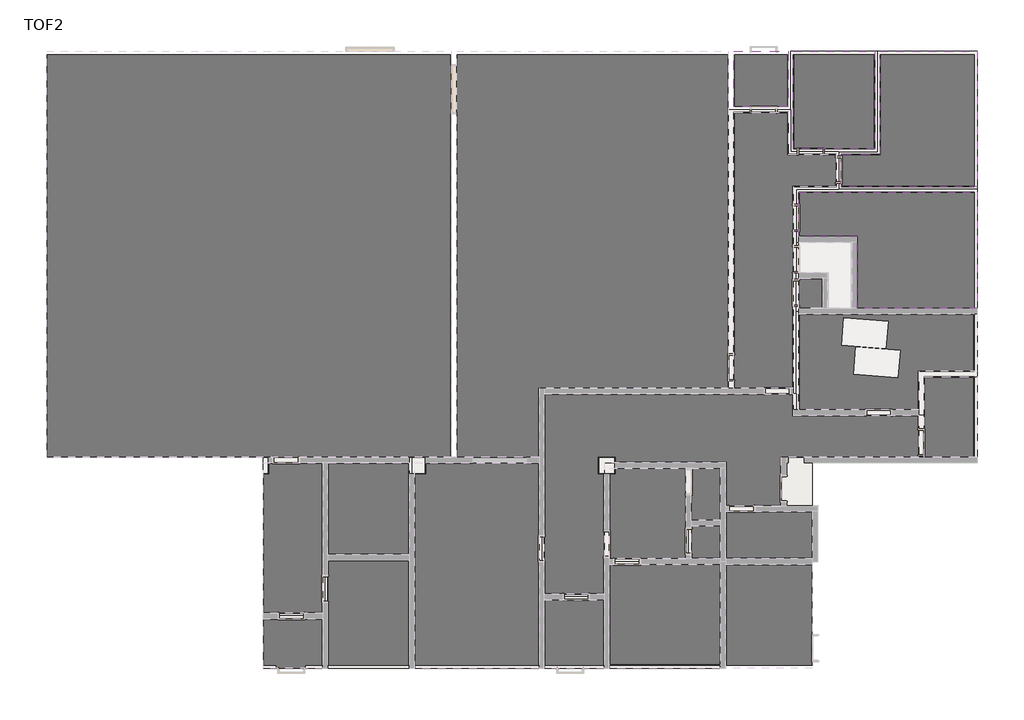
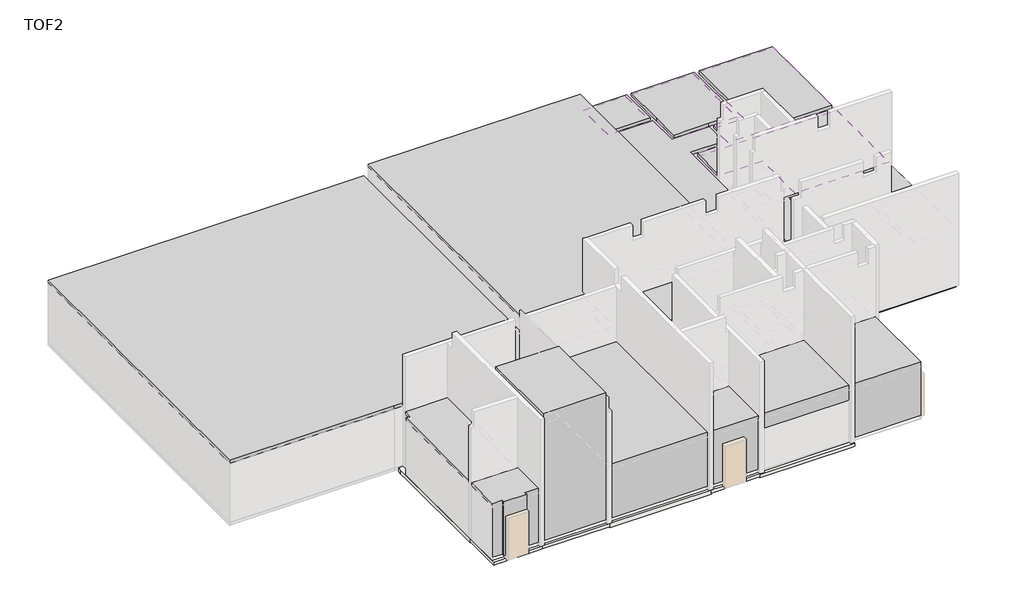
# One storey, part 5 of 5: 24 slabs, 23 proxies, 4 coverings.
# Revit data of these elements (continued)
# Type "H_FL_AR_B07_Vinyl Tile" (continued)
#   Description = ""
#   H_Q'ty Cal Type Tag = "FL-Q1"
#   Function = 0
#   Layers, outside or top first: 7 mm "Vinyl Composition Tile" (function 4)
# Elements 1, 2, 3, 4, 5, 6, 7, 8, 9, 10, 11, 12, 13, 14, 15, 16, 17, 18, 19, 20, 21, 22, 23 (IfcBuildingElementProxy)
#   Comments = "Room Check View Only"
#   Phase Created = New Construction
#   Materials on its faces: "Default"
# Elements 24, 25, 26, 27 (IfcCovering, "H_CE_AR_B09_Acoustic Ceiling_T Bar_600x600x9T")
#   Height Offset From Level = 2700 mm
#   Phase Created = New Construction
# Elements 28, 31, 42, 44, 45 (IfcSlab, "H_SF_AR_S17_SOG T200_GS1")
#   Height Offset From Level = 0 mm
#   Phase Created = New Construction
#   Materials on its faces: "Concrete - Cast-in-Place Concrete - 35 MPa"
# Elements 29, 30, 32, 33, 39 (IfcSlab, "H_SF_AR_S17_SOG T150_GS1")
#   Height Offset From Level = -50 mm
#   Phase Created = New Construction
#   Materials on its faces: "Concrete - Cast-in-Place Concrete - 35 MPa"
# Elements 34, 35, 36, 37, 38, 40, 41, 43, 46 (IfcSlab, "H_SF_AR_S17_SOG T150_GS1")
#   Height Offset From Level = 0 mm
#   Phase Created = New Construction
#   Materials on its faces: "Concrete - Cast-in-Place Concrete - 35 MPa"
# Elements 47, 48, 49, 50, 51 (IfcSlab, "H_FL_AR_B07_Vinyl Tile")
#   Height Offset From Level = 7 mm
#   Phase Created = New Construction
#   Materials on its faces: "Vinyl Composition Tile"
# Materials
#   "Concrete - Cast-in-Place Concrete - 35 MPa": class "Concrete", colour RGB 192 192 192, transparency 0, Description = "ACRYLIC EMULSION PAINT ON THK.13 CEMENT PLASTER", Cost = 0
#   "Vinyl Composition Tile": class "Generic", colour RGB 104 103 102, transparency 0, Description = "Vinyl Composition Tile", Cost = 0
#   "Default": class "Miscellaneous", colour RGB 80 80 80, transparency 0
# Room at (9390, 17931.521) mm, phase "New Construction", upper level "TOC", upper offset 2000 mm, lower offset -1000 mm
#   Comments = ""
#   Number = "101"
#   Name = "MECHANICAL ROOM"
#   H_Floor Finish Style Name = "Non-Slip Epoxy Paint"
#   H_Floor Base Material = "Concrete Slab / Steel Trowel Finish"
#   H_Wall-Base Material-1 = "Masonry Wall"
#   H_Skirt Finish Style Name = "Epoxy Paint"
#   H_Wall-Base Material-2 = ""
#   H_Wall-Base Material-3 = "Plastering"
#   H_Floor-Base Material-1 = "Concrete Slab"
#   H_Floor-Base Material-2 = "Steel Trowel Finish"
#   H_Floor-Base Material-3 = ""
#   H_Floor-Base Material-4 = ""
#   H_Floor-Base Material-5 = ""
#   H_Floor Finish-1 = "Epoxy Paint"
#   H_Floor Finish-2 = ""
#   H_Floor Finish Remark = "*WM 기준 확인 필요 Epoxy Paint \n(용제형, 0.1mm 이하) : epoxy resin + polyamine hardener(경화제)"
#   H_Skirt Base Material = "Same as Wall"
#   H_Skirt-Base Material-1 = ""
#   H_Skirt-Base Material-2 = ""
#   H_Skirt-Base Material-3 = ""
#   H_Skirt-Base Material-4 = ""
#   H_Skirt-Base Material-5 = ""
#   H_Skirt Finish-1 = "Epoxy Paint"
#   H_Skirt Finish-2 = ""
#   H_Skirt Finish Remark = "SACE"
#   H_Wall Finish Style Name = "Acrylic Emulsion Paint"
#   H_Wall Base Material = "Masonry Wall / Cement Plaster"
#   H_Wall-Base Material-4 = ""
#   H_Wall-Base Material-5 = ""
#   H_Wall Finish-1 = "Acrylic Emulsion Paint"
#   H_Wall Finish-2 = ""
#   H_Wall Finish Remark = "T13 Plaster"
#   H_Ceiling Finish Style Name = "Acrylic Emulsion Paint"
#   H_Ceiling Base Material = "Concrete Slab / Fair Faced Concrete"
#   H_Ceiling-Base Material-1 = "(Concrete Slab)"
#   H_Ceiling-Base Material-2 = ""
#   H_Ceiling-Base Material-3 = ""
#   H_Ceiling-Base Material-4 = ""
#   H_Ceiling-Base Material-5 = ""
#   H_Ceiling Finish-1 = "Acrylic Emulsion Paint"
#   H_Ceiling Finish-2 = ""
#   H_Ceiling Finish Remark = "SACE"
#   H_Room W = 17700 mm
#   H_Room L = 11400 mm
#   H_Room H or CH = 7300 mm
#   Floor Finish Style No = F06A
#   Skirt Finish Style No = B03
#   Wall Finish Style No = W01B
#   Ceiling Finish Style No = C01
# Room at (9390, 6347.521) mm, phase "New Construction", upper level "TOC", upper offset 2000 mm, lower offset -1000 mm
#   Comments = ""
#   Number = "112"
#   Name = "ELECTRICAL ROOM(SS08)"
#   H_Floor Finish Style Name = "Non-Slip Epoxy Paint"
#   H_Floor Base Material = "Concrete Slab / Screed"
#   H_Wall-Base Material-1 = "Masonry Wall"
#   H_Skirt Finish Style Name = "Epoxy Paint"
#   H_Wall-Base Material-2 = ""
#   H_Wall-Base Material-3 = "Plastering"
#   H_Floor-Base Material-1 = "Concrete Slab"
#   H_Floor-Base Material-2 = ""
#   H_Floor-Base Material-3 = "Screed"
#   H_Floor-Base Material-4 = ""
#   H_Floor-Base Material-5 = ""
#   H_Floor Finish-1 = "Epoxy Paint"
#   H_Floor Finish-2 = ""
#   H_Floor Finish Remark = "*WM 기준 확인 필요 Epoxy Paint \n(용제형, 0.1mm 이하) : epoxy resin + polyamine hardener(경화제)"
#   H_Skirt Base Material = "Same as Wall"
#   H_Skirt-Base Material-1 = ""
#   H_Skirt-Base Material-2 = ""
#   H_Skirt-Base Material-3 = ""
#   H_Skirt-Base Material-4 = ""
#   H_Skirt-Base Material-5 = ""
#   H_Skirt Finish-1 = "Epoxy Paint"
#   H_Skirt Finish-2 = ""
#   H_Skirt Finish Remark = "SACE"
#   H_Wall Finish Style Name = "Acrylic Emulsion Paint"
#   H_Wall Base Material = "Masonry Wall / Cement Plaster"
#   H_Wall-Base Material-4 = ""
#   H_Wall-Base Material-5 = ""
#   H_Wall Finish-1 = "Acrylic Emulsion Paint"
#   H_Wall Finish-2 = ""
#   H_Wall Finish Remark = "T13 Plaster"
#   H_Ceiling Finish Style Name = "Acrylic Emulsion Paint"
#   H_Ceiling Base Material = "Concrete Slab / Fair Faced Concrete"
#   H_Ceiling-Base Material-1 = "(Concrete Slab)"
#   H_Ceiling-Base Material-2 = ""
#   H_Ceiling-Base Material-3 = ""
#   H_Ceiling-Base Material-4 = ""
#   H_Ceiling-Base Material-5 = ""
#   H_Ceiling Finish-1 = "Acrylic Emulsion Paint"
#   H_Ceiling Finish-2 = ""
#   H_Ceiling Finish Remark = "SACE"
#   H_Room W = 17700 mm
#   H_Room L = 11000 mm
#   H_Room H or CH = 7300 mm
#   Floor Finish Style No = F06B
#   Skirt Finish Style No = B03
#   Wall Finish Style No = W01B
#   Ceiling Finish Style No = C01
# Room at (25850, 15981.521) mm, phase "New Construction", upper level "TOC", upper offset 2000 mm, lower offset 0 mm
#   Comments = ""
#   Number = "102"
#   Name = "RACK ROOM"
#   H_Floor Finish Style Name = "Anti-Dust Epoxy Paint / Anti-Static Vinyl Tile on Raised Floor"
#   H_Floor Base Material = "Concrete Slab / Steel Trowel Finish"
#   H_Wall-Base Material-1 = "Masonry Wall"
#   H_Skirt Finish Style Name = "Coved Vinyl Tile"
#   H_Wall-Base Material-2 = ""
#   H_Wall-Base Material-3 = "Plastering"
#   H_Floor-Base Material-1 = "Concrete Slab"
#   H_Floor-Base Material-2 = "Steel Trowel Finish"
#   H_Floor-Base Material-3 = ""
#   H_Floor-Base Material-4 = ""
#   H_Floor-Base Material-5 = "Raised Floor_Anti-Static Vinyl Tile"
#   H_Floor Finish-1 = "Anti-Dust Paint"
#   H_Floor Finish-2 = "Raised Floor_Anti-Static Vinyl Tile"
#   H_Floor Finish Remark = "600x600, H=1000"
#   H_Skirt Base Material = "Same as Wall"
#   H_Skirt-Base Material-1 = ""
#   H_Skirt-Base Material-2 = ""
#   H_Skirt-Base Material-3 = ""
#   H_Skirt-Base Material-4 = ""
#   H_Skirt-Base Material-5 = ""
#   H_Skirt Finish-1 = "Vinyl Tile"
#   H_Skirt Finish-2 = ""
#   H_Skirt Finish Remark = "Vinyl Tile = PVC Tile (polyvinyl chloride)"
#   H_Wall Finish Style Name = "Acrylic Emulsion Paint"
#   H_Wall Base Material = "Masonry Wall / Cement Plaster"
#   H_Wall-Base Material-4 = ""
#   H_Wall-Base Material-5 = ""
#   H_Wall Finish-1 = "Acrylic Emulsion Paint"
#   H_Wall Finish-2 = ""
#   H_Wall Finish Remark = "T13 Plaster"
#   H_Ceiling Finish Style Name = "Suspended Acoustic Tiled Ceiling (M-Bar)"
#   H_Ceiling Base Material = "Concrete Slab / Fair Faced Concrete"
#   H_Ceiling-Base Material-1 = "(Concrete Slab)"
#   H_Ceiling-Base Material-2 = "(Fair Faced Concrete)"
#   H_Ceiling-Base Material-3 = ""
#   H_Ceiling-Base Material-4 = ""
#   H_Ceiling-Base Material-5 = "Acoustic Tiled Ceiling System (M-Bar)"
#   H_Ceiling Finish-1 = "Acoustic Tiled Ceiling System (M-Bar)"
#   H_Ceiling Finish-2 = ""
#   H_Ceiling Finish Remark = ""
#   H_Room W = 14900 mm
#   H_Room L = 14900 mm
#   H_Room H or CH = 3000 mm
#   Floor Finish Style No = F91
#   Skirt Finish Style No = B35
#   Wall Finish Style No = W01B
#   Ceiling Finish Style No = C95A
# Room at (22100, 4784.521) mm, phase "New Construction", upper level "TOC", upper offset 2000 mm, lower offset -1000 mm
#   Comments = ""
#   Number = "114"
#   Name = "BATTERY ROOM"
#   H_Floor Finish Style Name = "Acid Resistant Ceramic Tile"
#   H_Floor Base Material = "Concrete Slab / Steel Trowel Finish"
#   H_Wall-Base Material-1 = "Masonry Wall"
#   H_Skirt Finish Style Name = "Coved Vinyl Tile"
#   H_Wall-Base Material-2 = ""
#   H_Wall-Base Material-3 = "Plastering"
#   H_Floor-Base Material-1 = "Concrete Slab"
#   H_Floor-Base Material-2 = "Steel Trowel Finish"
#   H_Floor-Base Material-3 = ""
#   H_Floor-Base Material-4 = ""
#   H_Floor-Base Material-5 = "Acid/Alkaline Resistant Tile"
#   H_Floor Finish-1 = "Acid/Alkaline Resistant Tile"
#   H_Floor Finish-2 = ""
#   H_Floor Finish Remark = "*WM : Bonding용 Mortar은 Tile에 포함\n*Slope 용 Screed만 별도 구분 (Concrete 바닥 단차 발생하는 경우 Only)"
#   H_Skirt Base Material = "Same as Wall"
#   H_Skirt-Base Material-1 = ""
#   H_Skirt-Base Material-2 = ""
#   H_Skirt-Base Material-3 = ""
#   H_Skirt-Base Material-4 = ""
#   H_Skirt-Base Material-5 = ""
#   H_Skirt Finish-1 = "Vinyl Tile"
#   H_Skirt Finish-2 = ""
#   H_Skirt Finish Remark = "Vinyl Tile = PVC Tile (polyvinyl chloride)"
#   H_Wall Finish Style Name = "Acid Resistant Paint"
#   H_Wall Base Material = "Masonry Wall / Cement Plaster"
#   H_Wall-Base Material-4 = ""
#   H_Wall-Base Material-5 = ""
#   H_Wall Finish-1 = "Acid/Alkaline Resistant Paint"
#   H_Wall Finish-2 = ""
#   H_Wall Finish Remark = "T13 Plaster"
#   H_Ceiling Finish Style Name = "Acrylic Emulsion Paint"
#   H_Ceiling Base Material = "Concrete Slab / Fair Faced Concrete"
#   H_Ceiling-Base Material-1 = "(Concrete Slab)"
#   H_Ceiling-Base Material-2 = ""
#   H_Ceiling-Base Material-3 = ""
#   H_Ceiling-Base Material-4 = ""
#   H_Ceiling-Base Material-5 = ""
#   H_Ceiling Finish-1 = "Acrylic Emulsion Paint"
#   H_Ceiling Finish-2 = ""
#   H_Ceiling Finish Remark = "SACE"
#   H_Room W = 7700 mm
#   H_Room L = 7500 mm
#   H_Room H or CH = 7300 mm
#   Floor Finish Style No = F32A
#   Skirt Finish Style No = B35
#   Wall Finish Style No = W04B
#   Ceiling Finish Style No = C01
# Room at (34305, 4784.521) mm, phase "New Construction", upper level "TOC", upper offset 2000 mm, lower offset 0 mm
#   Comments = ""
#   Number = "118"
#   Name = "DRIVERS LOUNGE"
#   H_Floor Finish Style Name = "Vinyl Tile"
#   H_Floor Base Material = "Concrete Slab / Steel Trowel Finish"
#   H_Wall-Base Material-1 = "Masonry Wall"
#   H_Skirt Finish Style Name = "Coved Vinyl Tile"
#   H_Wall-Base Material-2 = ""
#   H_Wall-Base Material-3 = "Plastering"
#   H_Floor-Base Material-1 = "Concrete Slab"
#   H_Floor-Base Material-2 = "Steel Trowel Finish"
#   H_Floor-Base Material-3 = ""
#   H_Floor-Base Material-4 = ""
#   H_Floor-Base Material-5 = "Vinyl Tile"
#   H_Floor Finish-1 = "Vinyl Tile"
#   H_Floor Finish-2 = ""
#   H_Floor Finish Remark = ""
#   H_Skirt Base Material = "Same as Wall"
#   H_Skirt-Base Material-1 = ""
#   H_Skirt-Base Material-2 = ""
#   H_Skirt-Base Material-3 = ""
#   H_Skirt-Base Material-4 = ""
#   H_Skirt-Base Material-5 = ""
#   H_Skirt Finish-1 = "Vinyl Tile"
#   H_Skirt Finish-2 = ""
#   H_Skirt Finish Remark = "Vinyl Tile = PVC Tile (polyvinyl chloride)"
#   H_Wall Finish Style Name = "Acrylic Emulsion Paint"
#   H_Wall Base Material = "Masonry Wall / Cement Plaster"
#   H_Wall-Base Material-4 = ""
#   H_Wall-Base Material-5 = ""
#   H_Wall Finish-1 = "Acrylic Emulsion Paint"
#   H_Wall Finish-2 = ""
#   H_Wall Finish Remark = "T13 Plaster"
#   H_Ceiling Finish Style Name = "Suspended Acoustic Tiled Ceiling (M-Bar)"
#   H_Ceiling Base Material = "Concrete Slab / Fair Faced Concrete"
#   H_Ceiling-Base Material-1 = "(Concrete Slab)"
#   H_Ceiling-Base Material-2 = "(Fair Faced Concrete)"
#   H_Ceiling-Base Material-3 = ""
#   H_Ceiling-Base Material-4 = ""
#   H_Ceiling-Base Material-5 = "Acoustic Tiled Ceiling System (M-Bar)"
#   H_Ceiling Finish-1 = "Acoustic Tiled Ceiling System (M-Bar)"
#   H_Ceiling Finish-2 = ""
#   H_Ceiling Finish Remark = ""
#   H_Room W = 4500 mm
#   H_Room L = 7500 mm
#   H_Room H or CH = 2600 mm
#   Floor Finish Style No = F34A
#   Skirt Finish Style No = B35
#   Wall Finish Style No = W01B
#   Ceiling Finish Style No = C95A
# Room at (38540.953, 16104.521) mm, phase "New Construction", upper level "TOC", upper offset 2000 mm, lower offset 0 mm
#   Comments = ""
#   Number = "103"
#   Name = "CONTROL ROOM"
#   H_Floor Finish Style Name = "Anti-Dust Epoxy Paint / Anti-Static Vinyl Tile on Raised Floor"
#   H_Floor Base Material = "Concrete Slab / Steel Trowel Finish"
#   H_Wall-Base Material-1 = "Masonry Wall"
#   H_Skirt Finish Style Name = "Coved Vinyl Tile"
#   H_Wall-Base Material-2 = ""
#   H_Wall-Base Material-3 = "Plastering"
#   H_Floor-Base Material-1 = "Concrete Slab"
#   H_Floor-Base Material-2 = "Steel Trowel Finish"
#   H_Floor-Base Material-3 = ""
#   H_Floor-Base Material-4 = ""
#   H_Floor-Base Material-5 = "Raised Floor_Anti-Static Vinyl Tile"
#   H_Floor Finish-1 = "Anti-Dust Paint"
#   H_Floor Finish-2 = "Raised Floor_Anti-Static Vinyl Tile"
#   H_Floor Finish Remark = "600x600, H=1000"
#   H_Skirt Base Material = "Same as Wall"
#   H_Skirt-Base Material-1 = ""
#   H_Skirt-Base Material-2 = ""
#   H_Skirt-Base Material-3 = ""
#   H_Skirt-Base Material-4 = ""
#   H_Skirt-Base Material-5 = ""
#   H_Skirt Finish-1 = "Vinyl Tile"
#   H_Skirt Finish-2 = ""
#   H_Skirt Finish Remark = "Vinyl Tile = PVC Tile (polyvinyl chloride)"
#   H_Wall Finish Style Name = "Acrylic Emulsion Paint"
#   H_Wall Base Material = "Masonry Wall / Cement Plaster"
#   H_Wall-Base Material-4 = ""
#   H_Wall-Base Material-5 = ""
#   H_Wall Finish-1 = "Acrylic Emulsion Paint"
#   H_Wall Finish-2 = ""
#   H_Wall Finish Remark = "T13 Plaster"
#   H_Ceiling Finish Style Name = "Suspended Acoustic Tiled Ceiling (M-Bar)"
#   H_Ceiling Base Material = "Concrete Slab / Fair Faced Concrete"
#   H_Ceiling-Base Material-1 = "(Concrete Slab)"
#   H_Ceiling-Base Material-2 = "(Fair Faced Concrete)"
#   H_Ceiling-Base Material-3 = ""
#   H_Ceiling-Base Material-4 = ""
#   H_Ceiling-Base Material-5 = "Acoustic Tiled Ceiling System (M-Bar)"
#   H_Ceiling Finish-1 = "Acoustic Tiled Ceiling System (M-Bar)"
#   H_Ceiling Finish-2 = ""
#   H_Ceiling Finish Remark = ""
#   H_Room W = 10000 mm
#   H_Room L = 14900 mm
#   H_Room H or CH = 3500 mm
#   Floor Finish Style No = F91
#   Skirt Finish Style No = B35
#   Wall Finish Style No = W01B
#   Ceiling Finish Style No = C95A
# Room at (41150, 2419.673) mm, phase "New Construction", upper level "TOC", upper offset 2000 mm, lower offset 0 mm
#   Comments = ""
#   Number = "122"
#   Name = "TOILETS"
#   H_Floor Finish Style Name = "Non-Slip Unglazed Ceramic Tile"
#   H_Floor Base Material = "Concrete Slab / Screed / Liquid Waterproofing"
#   H_Wall-Base Material-1 = "Masonry Wall"
#   H_Skirt Finish Style Name = "Coved Ceramic Tile"
#   H_Wall-Base Material-2 = ""
#   H_Wall-Base Material-3 = ""
#   H_Floor-Base Material-1 = "Concrete Slab"
#   H_Floor-Base Material-2 = ""
#   H_Floor-Base Material-3 = "Screed"
#   H_Floor-Base Material-4 = "Liquid Waterproofing"
#   H_Floor-Base Material-5 = "Ceramic Tile"
#   H_Floor Finish-1 = "Ceramic Tile"
#   H_Floor Finish-2 = ""
#   H_Floor Finish Remark = ""
#   H_Skirt Base Material = "Same as Wall"
#   H_Skirt-Base Material-1 = ""
#   H_Skirt-Base Material-2 = ""
#   H_Skirt-Base Material-3 = ""
#   H_Skirt-Base Material-4 = ""
#   H_Skirt-Base Material-5 = ""
#   H_Skirt Finish-1 = "Glazed Ceramic Tile"
#   H_Skirt Finish-2 = ""
#   H_Skirt Finish Remark = ""
#   H_Wall Finish Style Name = "Glazed Ceramic Tile (≤C.H+100) / No Paint (>C.H+100)"
#   H_Wall Base Material = "Masonry Wall / Liquid Waterproofing"
#   H_Wall-Base Material-4 = "Liquid Waterproofing"
#   H_Wall-Base Material-5 = "Glazed Ceramic Tile"
#   H_Wall Finish-1 = "Glazed Ceramic Tile"
#   H_Wall Finish-2 = ""
#   H_Wall Finish Remark = "Below Suspended Ceiling\nGlazed Ceramic Tile(≤C.H+100) + Liquid Waterproofing / No Paint (>C.H+100)"
#   H_Ceiling Finish Style Name = "Suspended Moisture Resistant Tiled Ceiling (M-Bar)"
#   H_Ceiling Base Material = "Concrete Slab / Fair Faced Concrete"
#   H_Ceiling-Base Material-1 = "(Concrete Slab)"
#   H_Ceiling-Base Material-2 = "(Fair Faced Concrete)"
#   H_Ceiling-Base Material-3 = ""
#   H_Ceiling-Base Material-4 = ""
#   H_Ceiling-Base Material-5 = "Moisture Resistant Tiled Ceiling System (M-Bar)"
#   H_Ceiling Finish-1 = "Moisture Resistant Tiled Ceiling System (M-Bar)"
#   H_Ceiling Finish-2 = ""
#   H_Ceiling Finish Remark = ""
#   H_Room W = 4000 mm
#   H_Room L = 3700 mm
#   H_Room H or CH = 2600 mm
#   Floor Finish Style No = F31B
#   Skirt Finish Style No = B32
#   Wall Finish Style No = W32B
#   Ceiling Finish Style No = C96A
# Room at (49742.5, 4429.521) mm, phase "New Construction", upper level "TOC", upper offset 2000 mm, lower offset -1000 mm
#   Comments = ""
#   Number = "125"
#   Name = "MAINTENANCE WORKSHOP"
#   H_Floor Finish Style Name = "Non-Slip Epoxy Paint"
#   H_Floor Base Material = "Concrete Slab / Steel Trowel Finish"
#   H_Wall-Base Material-1 = "Masonry Wall"
#   H_Skirt Finish Style Name = "Epoxy Paint"
#   H_Wall-Base Material-2 = ""
#   H_Wall-Base Material-3 = "Plastering"
#   H_Floor-Base Material-1 = "Concrete Slab"
#   H_Floor-Base Material-2 = "Steel Trowel Finish"
#   H_Floor-Base Material-3 = ""
#   H_Floor-Base Material-4 = ""
#   H_Floor-Base Material-5 = ""
#   H_Floor Finish-1 = "Epoxy Paint"
#   H_Floor Finish-2 = ""
#   H_Floor Finish Remark = "*WM 기준 확인 필요 Epoxy Paint \n(용제형, 0.1mm 이하) : epoxy resin + polyamine hardener(경화제)"
#   H_Skirt Base Material = "Same as Wall"
#   H_Skirt-Base Material-1 = ""
#   H_Skirt-Base Material-2 = ""
#   H_Skirt-Base Material-3 = ""
#   H_Skirt-Base Material-4 = ""
#   H_Skirt-Base Material-5 = ""
#   H_Skirt Finish-1 = "Epoxy Paint"
#   H_Skirt Finish-2 = ""
#   H_Skirt Finish Remark = "SACE"
#   H_Wall Finish Style Name = "Acrylic Emulsion Paint"
#   H_Wall Base Material = "Masonry Wall / Cement Plaster"
#   H_Wall-Base Material-4 = ""
#   H_Wall-Base Material-5 = ""
#   H_Wall Finish-1 = "Acrylic Emulsion Paint"
#   H_Wall Finish-2 = ""
#   H_Wall Finish Remark = "T13 Plaster"
#   H_Ceiling Finish Style Name = "Acrylic Emulsion Paint"
#   H_Ceiling Base Material = "Concrete Slab / Fair Faced Concrete"
#   H_Ceiling-Base Material-1 = "(Concrete Slab)"
#   H_Ceiling-Base Material-2 = ""
#   H_Ceiling-Base Material-3 = ""
#   H_Ceiling-Base Material-4 = ""
#   H_Ceiling-Base Material-5 = ""
#   H_Ceiling Finish-1 = "Acrylic Emulsion Paint"
#   H_Ceiling Finish-2 = ""
#   H_Ceiling Finish Remark = "SACE"
#   H_Room W = 6900 mm
#   H_Room L = 7500 mm
#   H_Room H or CH = 7300 mm
#   Floor Finish Style No = F06A
#   Skirt Finish Style No = B03
#   Wall Finish Style No = W01B
#   Ceiling Finish Style No = C01
# Room at (40470, 6702.369) mm, phase "New Construction", upper level "TOC", upper offset 2000 mm, lower offset 0 mm
#   Comments = ""
#   Number = "121"
#   Name = "LOCKER"
#   H_Floor Finish Style Name = "Non-Slip Unglazed Ceramic Tile"
#   H_Floor Base Material = "Concrete Slab / Steel Trowel Finish"
#   H_Wall-Base Material-1 = "Masonry Wall"
#   H_Skirt Finish Style Name = "Coved Ceramic Tile"
#   H_Wall-Base Material-2 = ""
#   H_Wall-Base Material-3 = ""
#   H_Floor-Base Material-1 = "Concrete Slab"
#   H_Floor-Base Material-2 = "Steel Trowel Finish"
#   H_Floor-Base Material-3 = ""
#   H_Floor-Base Material-4 = ""
#   H_Floor-Base Material-5 = "Ceramic Tile"
#   H_Floor Finish-1 = "Ceramic Tile"
#   H_Floor Finish-2 = ""
#   H_Floor Finish Remark = "*WM : Bonding용 Mortar은 Tile에 포함\n*Slope 용 Screed만 별도 구분 (Concrete 바닥 단차 발생하는 경우 Only)"
#   H_Skirt Base Material = "Same as Wall"
#   H_Skirt-Base Material-1 = ""
#   H_Skirt-Base Material-2 = ""
#   H_Skirt-Base Material-3 = ""
#   H_Skirt-Base Material-4 = ""
#   H_Skirt-Base Material-5 = ""
#   H_Skirt Finish-1 = "Glazed Ceramic Tile"
#   H_Skirt Finish-2 = ""
#   H_Skirt Finish Remark = ""
#   H_Wall Finish Style Name = "Glazed Ceramic Tile (≤C.H+100) / No Paint (>C.H+100)"
#   H_Wall Base Material = "Masonry Wall / Liquid Waterproofing"
#   H_Wall-Base Material-4 = "Liquid Waterproofing"
#   H_Wall-Base Material-5 = "Glazed Ceramic Tile"
#   H_Wall Finish-1 = "Glazed Ceramic Tile"
#   H_Wall Finish-2 = ""
#   H_Wall Finish Remark = "Below Suspended Ceiling\nGlazed Ceramic Tile(≤C.H+100) + Liquid Waterproofing / No Paint (>C.H+100)"
#   H_Ceiling Finish Style Name = "Suspended Moisture Resistant Tiled Ceiling (M-Bar)"
#   H_Ceiling Base Material = "Concrete Slab / Fair Faced Concrete"
#   H_Ceiling-Base Material-1 = "(Concrete Slab)"
#   H_Ceiling-Base Material-2 = "(Fair Faced Concrete)"
#   H_Ceiling-Base Material-3 = ""
#   H_Ceiling-Base Material-4 = ""
#   H_Ceiling-Base Material-5 = "Moisture Resistant Tiled Ceiling System (M-Bar)"
#   H_Ceiling Finish-1 = "Moisture Resistant Tiled Ceiling System (M-Bar)"
#   H_Ceiling Finish-2 = ""
#   H_Ceiling Finish Remark = ""
#   H_Room W = 2800 mm
#   H_Room L = 3300 mm
#   H_Room H or CH = 2700 mm
#   Floor Finish Style No = F31A
#   Skirt Finish Style No = B32
#   Wall Finish Style No = W32B
#   Ceiling Finish Style No = C96A
# Room at (42630, 7074.521) mm, phase "New Construction", upper level "TOC", upper offset 2000 mm, lower offset 0 mm
#   Comments = ""
#   Number = "127"
#   Name = "SHOWER ROOM"
#   H_Floor Finish Style Name = "Non-Slip Unglazed Ceramic Tile"
#   H_Floor Base Material = "Concrete Slab / Screed / Liquid Waterproofing"
#   H_Wall-Base Material-1 = "Concrete Wall"
#   H_Skirt Finish Style Name = "Epoxy Paint"
#   H_Wall-Base Material-2 = ""
#   H_Wall-Base Material-3 = ""
#   H_Floor-Base Material-1 = "Concrete Slab"
#   H_Floor-Base Material-2 = ""
#   H_Floor-Base Material-3 = "Screed"
#   H_Floor-Base Material-4 = "Liquid Waterproofing"
#   H_Floor-Base Material-5 = "Ceramic Tile"
#   H_Floor Finish-1 = "Ceramic Tile"
#   H_Floor Finish-2 = ""
#   H_Floor Finish Remark = ""
#   H_Skirt Base Material = "Same as Wall"
#   H_Skirt-Base Material-1 = ""
#   H_Skirt-Base Material-2 = ""
#   H_Skirt-Base Material-3 = ""
#   H_Skirt-Base Material-4 = ""
#   H_Skirt-Base Material-5 = ""
#   H_Skirt Finish-1 = "Epoxy Paint"
#   H_Skirt Finish-2 = ""
#   H_Skirt Finish Remark = "SACE"
#   H_Wall Finish Style Name = "Glazed Ceramic Tile (≤C.H+100) / No Paint (>C.H+100)"
#   H_Wall Base Material = "Concrete Wall"
#   H_Wall-Base Material-4 = "No Waterproofing"
#   H_Wall-Base Material-5 = "Glazed Ceramic Tile"
#   H_Wall Finish-1 = "Glazed Ceramic Tile"
#   H_Wall Finish-2 = ""
#   H_Wall Finish Remark = "Below Suspended Ceiling\nGlazed Ceramic Tile(≤C.H+100) / No Paint (>C.H+100)"
#   H_Ceiling Finish Style Name = "Suspended Moisture Resistant Tiled Ceiling (M-Bar)"
#   H_Ceiling Base Material = "Concrete Slab / Fair Faced Concrete"
#   H_Ceiling-Base Material-1 = "(Concrete Slab)"
#   H_Ceiling-Base Material-2 = "(Fair Faced Concrete)"
#   H_Ceiling-Base Material-3 = ""
#   H_Ceiling-Base Material-4 = ""
#   H_Ceiling-Base Material-5 = "Moisture Resistant Tiled Ceiling System (M-Bar)"
#   H_Ceiling Finish-1 = "Moisture Resistant Tiled Ceiling System (M-Bar)"
#   H_Ceiling Finish-2 = ""
#   H_Ceiling Finish Remark = ""
#   H_Room W = 1000 mm
#   H_Room L = 1900 mm
#   H_Room H or CH = 2600 mm
#   Floor Finish Style No = F31B
#   Skirt Finish Style No = B03
#   Wall Finish Style No = W32C
#   Ceiling Finish Style No = C96A
# Room at (42695, 5872.369) mm, phase "New Construction", upper level "TOC", upper offset 2000 mm, lower offset 0 mm
#   Comments = ""
#   Number = "128"
#   Name = "EWH ROOM"
#   H_Floor Finish Style Name = "Non-Slip Unglazed Ceramic Tile"
#   H_Floor Base Material = "Concrete Slab / Steel Trowel Finish"
#   H_Wall-Base Material-1 = "Masonry Wall"
#   H_Skirt Finish Style Name = "Epoxy Paint"
#   H_Wall-Base Material-2 = ""
#   H_Wall-Base Material-3 = "Plastering"
#   H_Floor-Base Material-1 = "Concrete Slab"
#   H_Floor-Base Material-2 = "Steel Trowel Finish"
#   H_Floor-Base Material-3 = ""
#   H_Floor-Base Material-4 = ""
#   H_Floor-Base Material-5 = "Ceramic Tile"
#   H_Floor Finish-1 = "Ceramic Tile"
#   H_Floor Finish-2 = ""
#   H_Floor Finish Remark = "*WM : Bonding용 Mortar은 Tile에 포함\n*Slope 용 Screed만 별도 구분 (Concrete 바닥 단차 발생하는 경우 Only)"
#   H_Skirt Base Material = "Same as Wall"
#   H_Skirt-Base Material-1 = ""
#   H_Skirt-Base Material-2 = ""
#   H_Skirt-Base Material-3 = ""
#   H_Skirt-Base Material-4 = ""
#   H_Skirt-Base Material-5 = ""
#   H_Skirt Finish-1 = "Epoxy Paint"
#   H_Skirt Finish-2 = ""
#   H_Skirt Finish Remark = "SACE"
#   H_Wall Finish Style Name = "Acrylic Emulsion Paint"
#   H_Wall Base Material = "Masonry Wall / Cement Plaster"
#   H_Wall-Base Material-4 = ""
#   H_Wall-Base Material-5 = ""
#   H_Wall Finish-1 = "Acrylic Emulsion Paint"
#   H_Wall Finish-2 = ""
#   H_Wall Finish Remark = "T13 Plaster"
#   H_Ceiling Finish Style Name = "Suspended Acoustic Tiled Ceiling (M-Bar)"
#   H_Ceiling Base Material = "Concrete Slab / Fair Faced Concrete"
#   H_Ceiling-Base Material-1 = "(Concrete Slab)"
#   H_Ceiling-Base Material-2 = "(Fair Faced Concrete)"
#   H_Ceiling-Base Material-3 = ""
#   H_Ceiling-Base Material-4 = ""
#   H_Ceiling-Base Material-5 = "Acoustic Tiled Ceiling System (M-Bar)"
#   H_Ceiling Finish-1 = "Acoustic Tiled Ceiling System (M-Bar)"
#   H_Ceiling Finish-2 = ""
#   H_Ceiling Finish Remark = ""
#   H_Room W = 1000 mm
#   H_Room L = 1200 mm
#   H_Room H or CH = 2700 mm
#   Floor Finish Style No = F31A
#   Skirt Finish Style No = B03
#   Wall Finish Style No = W01B
#   Ceiling Finish Style No = C95A
# Room at (52032, 10149.521) mm, phase "New Construction", upper level "TOC", upper offset 2000 mm, lower offset 0 mm
#   Comments = ""
#   Number = "110"
#   Name = "ABLUTIONS"
#   H_Floor Finish Style Name = "Non-Slip Unglazed Ceramic Tile"
#   H_Floor Base Material = "Concrete Slab / Screed / Liquid Waterproofing"
#   H_Wall-Base Material-1 = "Masonry Wall"
#   H_Skirt Finish Style Name = "Coved Ceramic Tile"
#   H_Wall-Base Material-2 = ""
#   H_Wall-Base Material-3 = ""
#   H_Floor-Base Material-1 = "Concrete Slab"
#   H_Floor-Base Material-2 = ""
#   H_Floor-Base Material-3 = "Screed"
#   H_Floor-Base Material-4 = "Liquid Waterproofing"
#   H_Floor-Base Material-5 = "Ceramic Tile"
#   H_Floor Finish-1 = "Ceramic Tile"
#   H_Floor Finish-2 = ""
#   H_Floor Finish Remark = ""
#   H_Skirt Base Material = "Same as Wall"
#   H_Skirt-Base Material-1 = ""
#   H_Skirt-Base Material-2 = ""
#   H_Skirt-Base Material-3 = ""
#   H_Skirt-Base Material-4 = ""
#   H_Skirt-Base Material-5 = ""
#   H_Skirt Finish-1 = "Glazed Ceramic Tile"
#   H_Skirt Finish-2 = ""
#   H_Skirt Finish Remark = ""
#   H_Wall Finish Style Name = "Glazed Ceramic Tile (≤C.H+100) / No Paint (>C.H+100)"
#   H_Wall Base Material = "Masonry Wall / Liquid Waterproofing"
#   H_Wall-Base Material-4 = "Liquid Waterproofing"
#   H_Wall-Base Material-5 = "Glazed Ceramic Tile"
#   H_Wall Finish-1 = "Glazed Ceramic Tile"
#   H_Wall Finish-2 = ""
#   H_Wall Finish Remark = "Below Suspended Ceiling\nGlazed Ceramic Tile(≤C.H+100) + Liquid Waterproofing / No Paint (>C.H+100)"
#   H_Ceiling Finish Style Name = "Suspended Moisture Resistant Tiled Ceiling (M-Bar)"
#   H_Ceiling Base Material = "Concrete Slab / Fair Faced Concrete"
#   H_Ceiling-Base Material-1 = "(Concrete Slab)"
#   H_Ceiling-Base Material-2 = "(Fair Faced Concrete)"
#   H_Ceiling-Base Material-3 = ""
#   H_Ceiling-Base Material-4 = ""
#   H_Ceiling-Base Material-5 = "Moisture Resistant Tiled Ceiling System (M-Bar)"
#   H_Ceiling Finish-1 = "Moisture Resistant Tiled Ceiling System (M-Bar)"
#   H_Ceiling Finish-2 = ""
#   H_Ceiling Finish Remark = ""
#   H_Room W = 1800 mm
#   H_Room L = 2900 mm
#   H_Room H or CH = 2600 mm
#   Floor Finish Style No = F31B
#   Skirt Finish Style No = B32
#   Wall Finish Style No = W32B
#   Ceiling Finish Style No = C96A
# Room at (50280, 21414.521) mm, phase "New Construction", upper level "TOC", upper offset 2000 mm, lower offset 0 mm
#   Comments = ""
#   Number = "106"
#   Name = "SHIFT SUPERVISOR/DAY SUPERVISOR"
#   H_Floor Finish Style Name = "Vinyl Tile"
#   H_Floor Base Material = "Concrete Slab / Steel Trowel Finish"
#   H_Wall-Base Material-1 = "Masonry Wall"
#   H_Skirt Finish Style Name = "Coved Vinyl Tile"
#   H_Wall-Base Material-2 = ""
#   H_Wall-Base Material-3 = "Plastering"
#   H_Floor-Base Material-1 = "Concrete Slab"
#   H_Floor-Base Material-2 = "Steel Trowel Finish"
#   H_Floor-Base Material-3 = ""
#   H_Floor-Base Material-4 = ""
#   H_Floor-Base Material-5 = "Vinyl Tile"
#   H_Floor Finish-1 = "Vinyl Tile"
#   H_Floor Finish-2 = ""
#   H_Floor Finish Remark = ""
#   H_Skirt Base Material = "Same as Wall"
#   H_Skirt-Base Material-1 = ""
#   H_Skirt-Base Material-2 = ""
#   H_Skirt-Base Material-3 = ""
#   H_Skirt-Base Material-4 = ""
#   H_Skirt-Base Material-5 = ""
#   H_Skirt Finish-1 = "Vinyl Tile"
#   H_Skirt Finish-2 = ""
#   H_Skirt Finish Remark = "Vinyl Tile = PVC Tile (polyvinyl chloride)"
#   H_Wall Finish Style Name = "Acrylic Emulsion Paint"
#   H_Wall Base Material = "Masonry Wall / Cement Plaster"
#   H_Wall-Base Material-4 = ""
#   H_Wall-Base Material-5 = ""
#   H_Wall Finish-1 = "Acrylic Emulsion Paint"
#   H_Wall Finish-2 = ""
#   H_Wall Finish Remark = "T13 Plaster"
#   H_Ceiling Finish Style Name = "Suspended Acoustic Tiled Ceiling (M-Bar)"
#   H_Ceiling Base Material = "Concrete Slab / Fair Faced Concrete"
#   H_Ceiling-Base Material-1 = "(Concrete Slab)"
#   H_Ceiling-Base Material-2 = "(Fair Faced Concrete)"
#   H_Ceiling-Base Material-3 = ""
#   H_Ceiling-Base Material-4 = ""
#   H_Ceiling-Base Material-5 = "Acoustic Tiled Ceiling System (M-Bar)"
#   H_Ceiling Finish-1 = "Acoustic Tiled Ceiling System (M-Bar)"
#   H_Ceiling Finish-2 = ""
#   H_Ceiling Finish Remark = ""
#   H_Room W = 4900 mm
#   H_Room L = 4900 mm
#   H_Room H or CH = 2600 mm
#   Floor Finish Style No = F34A
#   Skirt Finish Style No = B35
#   Wall Finish Style No = W01B
#   Ceiling Finish Style No = C95A
# Room at (44795, 22494.021) mm, phase "New Construction", upper level "TOC", upper offset 2000 mm, lower offset 0 mm
#   Comments = ""
#   Number = "104"
#   Name = "AIR LOCK"
#   H_Floor Finish Style Name = "Vinyl Tile"
#   H_Floor Base Material = "Concrete Slab / Steel Trowel Finish"
#   H_Wall-Base Material-1 = "Masonry Wall"
#   H_Skirt Finish Style Name = "Coved Vinyl Tile"
#   H_Wall-Base Material-2 = ""
#   H_Wall-Base Material-3 = "Plastering"
#   H_Floor-Base Material-1 = "Concrete Slab"
#   H_Floor-Base Material-2 = "Steel Trowel Finish"
#   H_Floor-Base Material-3 = ""
#   H_Floor-Base Material-4 = ""
#   H_Floor-Base Material-5 = "Vinyl Tile"
#   H_Floor Finish-1 = "Vinyl Tile"
#   H_Floor Finish-2 = ""
#   H_Floor Finish Remark = ""
#   H_Skirt Base Material = "Same as Wall"
#   H_Skirt-Base Material-1 = ""
#   H_Skirt-Base Material-2 = ""
#   H_Skirt-Base Material-3 = ""
#   H_Skirt-Base Material-4 = ""
#   H_Skirt-Base Material-5 = ""
#   H_Skirt Finish-1 = "Vinyl Tile"
#   H_Skirt Finish-2 = ""
#   H_Skirt Finish Remark = "Vinyl Tile = PVC Tile (polyvinyl chloride)"
#   H_Wall Finish Style Name = "Acrylic Emulsion Paint"
#   H_Wall Base Material = "Masonry Wall / Cement Plaster"
#   H_Wall-Base Material-4 = ""
#   H_Wall-Base Material-5 = ""
#   H_Wall Finish-1 = "Acrylic Emulsion Paint"
#   H_Wall Finish-2 = ""
#   H_Wall Finish Remark = "T13 Plaster"
#   H_Ceiling Finish Style Name = "Suspended Acoustic Tiled Ceiling (M-Bar)"
#   H_Ceiling Base Material = "Concrete Slab / Fair Faced Concrete"
#   H_Ceiling-Base Material-1 = "(Concrete Slab)"
#   H_Ceiling-Base Material-2 = "(Fair Faced Concrete)"
#   H_Ceiling-Base Material-3 = ""
#   H_Ceiling-Base Material-4 = ""
#   H_Ceiling-Base Material-5 = "Acoustic Tiled Ceiling System (M-Bar)"
#   H_Ceiling Finish-1 = "Acoustic Tiled Ceiling System (M-Bar)"
#   H_Ceiling Finish-2 = ""
#   H_Ceiling Finish Remark = ""
#   H_Room W = 1900 mm
#   H_Room L = 1900 mm
#   H_Room H or CH = 2600 mm
#   Floor Finish Style No = F34A
#   Skirt Finish Style No = B35
#   Wall Finish Style No = W01B
#   Ceiling Finish Style No = C95A
# Room at (45465, 16437.021) mm, phase "New Construction", upper level "TOC", upper offset 2000 mm, lower offset 0 mm
#   Comments = ""
#   Number = "107"
#   Name = "CORRIDOR"
#   H_Floor Finish Style Name = "Vinyl Tile"
#   H_Floor Base Material = "Concrete Slab / Steel Trowel Finish"
#   H_Wall-Base Material-1 = "Masonry Wall"
#   H_Skirt Finish Style Name = "Coved Vinyl Tile"
#   H_Wall-Base Material-2 = ""
#   H_Wall-Base Material-3 = "Plastering"
#   H_Floor-Base Material-1 = "Concrete Slab"
#   H_Floor-Base Material-2 = "Steel Trowel Finish"
#   H_Floor-Base Material-3 = ""
#   H_Floor-Base Material-4 = ""
#   H_Floor-Base Material-5 = "Vinyl Tile"
#   H_Floor Finish-1 = "Vinyl Tile"
#   H_Floor Finish-2 = ""
#   H_Floor Finish Remark = ""
#   H_Skirt Base Material = "Same as Wall"
#   H_Skirt-Base Material-1 = ""
#   H_Skirt-Base Material-2 = ""
#   H_Skirt-Base Material-3 = ""
#   H_Skirt-Base Material-4 = ""
#   H_Skirt-Base Material-5 = ""
#   H_Skirt Finish-1 = "Vinyl Tile"
#   H_Skirt Finish-2 = ""
#   H_Skirt Finish Remark = "Vinyl Tile = PVC Tile (polyvinyl chloride)"
#   H_Wall Finish Style Name = "Acrylic Emulsion Paint"
#   H_Wall Base Material = "Masonry Wall / Cement Plaster"
#   H_Wall-Base Material-4 = ""
#   H_Wall-Base Material-5 = ""
#   H_Wall Finish-1 = "Acrylic Emulsion Paint"
#   H_Wall Finish-2 = ""
#   H_Wall Finish Remark = "T13 Plaster"
#   H_Ceiling Finish Style Name = "Suspended Acoustic Tiled Ceiling (M-Bar)"
#   H_Ceiling Base Material = "Concrete Slab / Fair Faced Concrete"
#   H_Ceiling-Base Material-1 = "(Concrete Slab)"
#   H_Ceiling-Base Material-2 = "(Fair Faced Concrete)"
#   H_Ceiling-Base Material-3 = ""
#   H_Ceiling-Base Material-4 = ""
#   H_Ceiling-Base Material-5 = "Acoustic Tiled Ceiling System (M-Bar)"
#   H_Ceiling Finish-1 = "Acoustic Tiled Ceiling System (M-Bar)"
#   H_Ceiling Finish-2 = ""
#   H_Ceiling Finish Remark = ""
#   H_Room W = 3700 mm
#   H_Room L = 10100 mm
#   H_Room H or CH = 2600 mm
#   Floor Finish Style No = F34A
#   Skirt Finish Style No = B35
#   Wall Finish Style No = W01B
#   Ceiling Finish Style No = C95A
# Room at (47300, 21676.521) mm, phase "New Construction", upper level "TOC", upper offset 2000 mm, lower offset 0 mm
#   Comments = ""
#   Number = "105"
#   Name = "LIBRARY"
#   H_Floor Finish Style Name = "Vinyl Tile"
#   H_Floor Base Material = "Concrete Slab / Steel Trowel Finish"
#   H_Wall-Base Material-1 = "Masonry Wall"
#   H_Skirt Finish Style Name = "Coved Vinyl Tile"
#   H_Wall-Base Material-2 = ""
#   H_Wall-Base Material-3 = "Plastering"
#   H_Floor-Base Material-1 = "Concrete Slab"
#   H_Floor-Base Material-2 = "Steel Trowel Finish"
#   H_Floor-Base Material-3 = ""
#   H_Floor-Base Material-4 = ""
#   H_Floor-Base Material-5 = "Vinyl Tile"
#   H_Floor Finish-1 = "Vinyl Tile"
#   H_Floor Finish-2 = ""
#   H_Floor Finish Remark = ""
#   H_Skirt Base Material = "Same as Wall"
#   H_Skirt-Base Material-1 = ""
#   H_Skirt-Base Material-2 = ""
#   H_Skirt-Base Material-3 = ""
#   H_Skirt-Base Material-4 = ""
#   H_Skirt-Base Material-5 = ""
#   H_Skirt Finish-1 = "Vinyl Tile"
#   H_Skirt Finish-2 = ""
#   H_Skirt Finish Remark = "Vinyl Tile = PVC Tile (polyvinyl chloride)"
#   H_Wall Finish Style Name = "Acrylic Emulsion Paint"
#   H_Wall Base Material = "Masonry Wall / Cement Plaster"
#   H_Wall-Base Material-4 = ""
#   H_Wall-Base Material-5 = ""
#   H_Wall Finish-1 = "Acrylic Emulsion Paint"
#   H_Wall Finish-2 = ""
#   H_Wall Finish Remark = "T13 Plaster"
#   H_Ceiling Finish Style Name = "Suspended Acoustic Tiled Ceiling (M-Bar)"
#   H_Ceiling Base Material = "Concrete Slab / Fair Faced Concrete"
#   H_Ceiling-Base Material-1 = "(Concrete Slab)"
#   H_Ceiling-Base Material-2 = "(Fair Faced Concrete)"
#   H_Ceiling-Base Material-3 = ""
#   H_Ceiling-Base Material-4 = ""
#   H_Ceiling-Base Material-5 = "Acoustic Tiled Ceiling System (M-Bar)"
#   H_Ceiling Finish-1 = "Acoustic Tiled Ceiling System (M-Bar)"
#   H_Ceiling Finish-2 = ""
#   H_Ceiling Finish Remark = ""
#   H_Room W = 2900 mm
#   H_Room L = 3500 mm
#   H_Room H or CH = 2600 mm
#   Floor Finish Style No = F34A
#   Skirt Finish Style No = B35
#   Wall Finish Style No = W01B
#   Ceiling Finish Style No = C95A
# Room at (49372, 12124.521) mm, phase "New Construction", upper level "TOC", upper offset 2000 mm, lower offset 0 mm
#   Comments = ""
#   Number = "111"
#   Name = "PRAYER ROOM"
#   H_Floor Finish Style Name = "Carpet Tile"
#   H_Floor Base Material = "Concrete Slab / Steel Trowel Finish"
#   H_Wall-Base Material-1 = "Masonry Wall"
#   H_Skirt Finish Style Name = "Coved Vinyl Tile"
#   H_Wall-Base Material-2 = ""
#   H_Wall-Base Material-3 = "Plastering"
#   H_Floor-Base Material-1 = "Concrete Slab"
#   H_Floor-Base Material-2 = ""
#   H_Floor-Base Material-3 = "Screed"
#   H_Floor-Base Material-5 = "Carpet Tile"
#   H_Floor Finish-1 = "Carpet Tile"
#   H_Skirt Base Material = "Same as Wall"
#   H_Skirt-Base Material-1 = ""
#   H_Skirt-Base Material-2 = ""
#   H_Skirt-Base Material-3 = ""
#   H_Skirt-Base Material-4 = ""
#   H_Skirt-Base Material-5 = ""
#   H_Skirt Finish-1 = "Vinyl Tile"
#   H_Skirt Finish-2 = ""
#   H_Skirt Finish Remark = "Vinyl Tile = PVC Tile (polyvinyl chloride)"
#   H_Wall Finish Style Name = "Acrylic Emulsion Paint"
#   H_Wall Base Material = "Masonry Wall / Cement Plaster"
#   H_Wall-Base Material-4 = ""
#   H_Wall-Base Material-5 = ""
#   H_Wall Finish-1 = "Acrylic Emulsion Paint"
#   H_Wall Finish-2 = ""
#   H_Wall Finish Remark = "T13 Plaster"
#   H_Ceiling Finish Style Name = "Suspended Acoustic Tiled Ceiling (M-Bar)"
#   H_Ceiling Base Material = "Concrete Slab / Fair Faced Concrete"
#   H_Ceiling-Base Material-1 = "(Concrete Slab)"
#   H_Ceiling-Base Material-2 = "(Fair Faced Concrete)"
#   H_Ceiling-Base Material-3 = ""
#   H_Ceiling-Base Material-4 = ""
#   H_Ceiling-Base Material-5 = "Acoustic Tiled Ceiling System (M-Bar)"
#   H_Ceiling Finish-1 = "Acoustic Tiled Ceiling System (M-Bar)"
#   H_Ceiling Finish-2 = ""
#   H_Ceiling Finish Remark = ""
#   H_Room W = 6400 mm
#   H_Room L = 3500 mm
#   H_Room H or CH = 2600 mm
#   Floor Finish Style No = F43-1
#   Skirt Finish Style No = B35
#   Wall Finish Style No = W01B
#   Ceiling Finish Style No = C95A
# Room at (49620, 16249.521) mm, phase "New Construction", upper level "TOC", upper offset 2000 mm, lower offset 0 mm
#   Comments = ""
#   Number = "108"
#   Name = "BREAK ROOM"
#   H_Floor Finish Style Name = "Vinyl Tile"
#   H_Floor Base Material = "Concrete Slab / Steel Trowel Finish"
#   H_Wall-Base Material-1 = "Masonry Wall"
#   H_Skirt Finish Style Name = "Coved Vinyl Tile"
#   H_Wall-Base Material-2 = ""
#   H_Wall-Base Material-3 = "Plastering"
#   H_Floor-Base Material-1 = "Concrete Slab"
#   H_Floor-Base Material-2 = "Steel Trowel Finish"
#   H_Floor-Base Material-3 = ""
#   H_Floor-Base Material-4 = ""
#   H_Floor-Base Material-5 = "Vinyl Tile"
#   H_Floor Finish-1 = "Vinyl Tile"
#   H_Floor Finish-2 = ""
#   H_Floor Finish Remark = ""
#   H_Skirt Base Material = "Same as Wall"
#   H_Skirt-Base Material-1 = ""
#   H_Skirt-Base Material-2 = ""
#   H_Skirt-Base Material-3 = ""
#   H_Skirt-Base Material-4 = ""
#   H_Skirt-Base Material-5 = ""
#   H_Skirt Finish-1 = "Vinyl Tile"
#   H_Skirt Finish-2 = ""
#   H_Skirt Finish Remark = "Vinyl Tile = PVC Tile (polyvinyl chloride)"
#   H_Wall Finish Style Name = "Acrylic Emulsion Paint"
#   H_Wall Base Material = "Masonry Wall / Cement Plaster"
#   H_Wall-Base Material-4 = ""
#   H_Wall-Base Material-5 = ""
#   H_Wall Finish-1 = "Acrylic Emulsion Paint"
#   H_Wall Finish-2 = ""
#   H_Wall Finish Remark = "T13 Plaster"
#   H_Ceiling Finish Style Name = "Suspended Moisture Resistant Tiled Ceiling (M-Bar)"
#   H_Ceiling Base Material = "Concrete Slab / Fair Faced Concrete"
#   H_Ceiling-Base Material-1 = "(Concrete Slab)"
#   H_Ceiling-Base Material-2 = "(Fair Faced Concrete)"
#   H_Ceiling-Base Material-3 = ""
#   H_Ceiling-Base Material-4 = ""
#   H_Ceiling-Base Material-5 = "Moisture Resistant Tiled Ceiling System (M-Bar)"
#   H_Ceiling Finish-1 = "Moisture Resistant Tiled Ceiling System (M-Bar)"
#   H_Ceiling Finish-2 = ""
#   H_Ceiling Finish Remark = ""
#   H_Room W = 6500 mm
#   H_Room L = 4200 mm
#   H_Room H or CH = 2600 mm
#   Floor Finish Style No = F34A
#   Skirt Finish Style No = B35
#   Wall Finish Style No = W01B
#   Ceiling Finish Style No = C96A
# Room at (47491.607, 15338.043) mm, phase "New Construction", upper level "TOC", upper offset 2000 mm, lower offset 0 mm
#   Comments = ""
#   Number = "109"
#   Name = "JANITOR"
#   H_Floor Finish Style Name = "Non-Slip Unglazed Ceramic Tile"
#   H_Floor Base Material = "Concrete Slab / Screed / Liquid Waterproofing"
#   H_Wall-Base Material-1 = "Masonry Wall"
#   H_Skirt Finish Style Name = "Coved Ceramic Tile"
#   H_Wall-Base Material-2 = ""
#   H_Wall-Base Material-3 = ""
#   H_Floor-Base Material-1 = "Concrete Slab"
#   H_Floor-Base Material-2 = ""
#   H_Floor-Base Material-3 = "Screed"
#   H_Floor-Base Material-4 = "Liquid Waterproofing"
#   H_Floor-Base Material-5 = "Ceramic Tile"
#   H_Floor Finish-1 = "Ceramic Tile"
#   H_Floor Finish-2 = ""
#   H_Floor Finish Remark = ""
#   H_Skirt Base Material = "Same as Wall"
#   H_Skirt-Base Material-1 = ""
#   H_Skirt-Base Material-2 = ""
#   H_Skirt-Base Material-3 = ""
#   H_Skirt-Base Material-4 = ""
#   H_Skirt-Base Material-5 = ""
#   H_Skirt Finish-1 = "Glazed Ceramic Tile"
#   H_Skirt Finish-2 = ""
#   H_Skirt Finish Remark = ""
#   H_Wall Finish Style Name = "Glazed Ceramic Tile (≤C.H+100) / No Paint (>C.H+100)"
#   H_Wall Base Material = "Masonry Wall / Liquid Waterproofing"
#   H_Wall-Base Material-4 = "Liquid Waterproofing"
#   H_Wall-Base Material-5 = "Glazed Ceramic Tile"
#   H_Wall Finish-1 = "Glazed Ceramic Tile"
#   H_Wall Finish-2 = ""
#   H_Wall Finish Remark = "Below Suspended Ceiling\nGlazed Ceramic Tile(≤C.H+100) + Liquid Waterproofing / No Paint (>C.H+100)"
#   H_Ceiling Finish Style Name = "Suspended Moisture Resistant Tiled Ceiling (M-Bar)"
#   H_Ceiling Base Material = "Concrete Slab / Fair Faced Concrete"
#   H_Ceiling-Base Material-1 = "(Concrete Slab)"
#   H_Ceiling-Base Material-2 = "(Fair Faced Concrete)"
#   H_Ceiling-Base Material-3 = ""
#   H_Ceiling-Base Material-4 = ""
#   H_Ceiling-Base Material-5 = "Moisture Resistant Tiled Ceiling System (M-Bar)"
#   H_Ceiling Finish-1 = "Moisture Resistant Tiled Ceiling System (M-Bar)"
#   H_Ceiling Finish-2 = ""
#   H_Ceiling Finish Remark = ""
#   H_Room W = 800 mm
#   H_Room L = 1100 mm
#   H_Room H or CH = 2600 mm
#   Floor Finish Style No = F31B
#   Skirt Finish Style No = B32
#   Wall Finish Style No = W32B
#   Ceiling Finish Style No = C96A
# Room at (46580, 14657.021) mm, phase "New Construction", upper level "TOC", upper offset 2000 mm, lower offset 0 mm
#   Comments = ""
#   Number = "126"
#   Name = "EWH ROOM"
#   H_Floor Finish Style Name = "Vinyl Tile"
#   H_Floor Base Material = "Concrete Slab / Steel Trowel Finish"
#   H_Wall-Base Material-1 = "Masonry Wall"
#   H_Skirt Finish Style Name = "Coved Vinyl Tile"
#   H_Wall-Base Material-2 = ""
#   H_Wall-Base Material-3 = "Plastering"
#   H_Floor-Base Material-1 = "Concrete Slab"
#   H_Floor-Base Material-2 = "Steel Trowel Finish"
#   H_Floor-Base Material-3 = ""
#   H_Floor-Base Material-4 = ""
#   H_Floor-Base Material-5 = "Vinyl Tile"
#   H_Floor Finish-1 = "Vinyl Tile"
#   H_Floor Finish-2 = ""
#   H_Floor Finish Remark = ""
#   H_Skirt Base Material = "Same as Wall"
#   H_Skirt-Base Material-1 = ""
#   H_Skirt-Base Material-2 = ""
#   H_Skirt-Base Material-3 = ""
#   H_Skirt-Base Material-4 = ""
#   H_Skirt-Base Material-5 = ""
#   H_Skirt Finish-1 = "Vinyl Tile"
#   H_Skirt Finish-2 = ""
#   H_Skirt Finish Remark = "Vinyl Tile = PVC Tile (polyvinyl chloride)"
#   H_Wall Finish Style Name = "Acrylic Emulsion Paint"
#   H_Wall Base Material = "Masonry Wall / Cement Plaster"
#   H_Wall-Base Material-4 = ""
#   H_Wall-Base Material-5 = ""
#   H_Wall Finish-1 = "Acrylic Emulsion Paint"
#   H_Wall Finish-2 = ""
#   H_Wall Finish Remark = "T13 Plaster"
#   H_Ceiling Finish Style Name = "Suspended Acoustic Tiled Ceiling (M-Bar)"
#   H_Ceiling Base Material = "Concrete Slab / Fair Faced Concrete"
#   H_Ceiling-Base Material-1 = "(Concrete Slab)"
#   H_Ceiling-Base Material-2 = "(Fair Faced Concrete)"
#   H_Ceiling-Base Material-3 = ""
#   H_Ceiling-Base Material-4 = ""
#   H_Ceiling-Base Material-5 = "Acoustic Tiled Ceiling System (M-Bar)"
#   H_Ceiling Finish-1 = "Acoustic Tiled Ceiling System (M-Bar)"
#   H_Ceiling Finish-2 = ""
#   H_Ceiling Finish Remark = ""
#   H_Room W = 3100 mm
#   H_Room L = 1700 mm
#   H_Room H or CH = 2600 mm
#   Floor Finish Style No = F34A
#   Skirt Finish Style No = B35
#   Wall Finish Style No = W01B
#   Ceiling Finish Style No = C95A
# Room at (45350, 5729.521) mm, phase "New Construction", upper level "TOC", upper offset 2000 mm, lower offset 0 mm
#   Comments = ""
#   Number = "123"
#   Name = "STORE"
#   H_Floor Finish Style Name = "Vinyl Tile"
#   H_Floor Base Material = "Concrete Slab / Steel Trowel Finish"
#   H_Wall-Base Material-1 = "Masonry Wall"
#   H_Skirt Finish Style Name = "Coved Vinyl Tile"
#   H_Wall-Base Material-2 = ""
#   H_Wall-Base Material-3 = "Plastering"
#   H_Floor-Base Material-1 = "Concrete Slab"
#   H_Floor-Base Material-2 = "Steel Trowel Finish"
#   H_Floor-Base Material-3 = ""
#   H_Floor-Base Material-4 = ""
#   H_Floor-Base Material-5 = "Vinyl Tile"
#   H_Floor Finish-1 = "Vinyl Tile"
#   H_Floor Finish-2 = ""
#   H_Floor Finish Remark = ""
#   H_Skirt Base Material = "Same as Wall"
#   H_Skirt-Base Material-1 = ""
#   H_Skirt-Base Material-2 = ""
#   H_Skirt-Base Material-3 = ""
#   H_Skirt-Base Material-4 = ""
#   H_Skirt-Base Material-5 = ""
#   H_Skirt Finish-1 = "Vinyl Tile"
#   H_Skirt Finish-2 = ""
#   H_Skirt Finish Remark = "Vinyl Tile = PVC Tile (polyvinyl chloride)"
#   H_Wall Finish Style Name = "Acrylic Emulsion Paint"
#   H_Wall Base Material = "Masonry Wall / Cement Plaster"
#   H_Wall-Base Material-4 = ""
#   H_Wall-Base Material-5 = ""
#   H_Wall Finish-1 = "Acrylic Emulsion Paint"
#   H_Wall Finish-2 = ""
#   H_Wall Finish Remark = "T13 Plaster"
#   H_Ceiling Finish Style Name = "Suspended Acoustic Tiled Ceiling (M-Bar)"
#   H_Ceiling Base Material = "Concrete Slab / Fair Faced Concrete"
#   H_Ceiling-Base Material-1 = "(Concrete Slab)"
#   H_Ceiling-Base Material-2 = "(Fair Faced Concrete)"
#   H_Ceiling-Base Material-3 = ""
#   H_Ceiling-Base Material-4 = ""
#   H_Ceiling-Base Material-5 = "Acoustic Tiled Ceiling System (M-Bar)"
#   H_Ceiling Finish-1 = "Acoustic Tiled Ceiling System (M-Bar)"
#   H_Ceiling Finish-2 = ""
#   H_Ceiling Finish Remark = ""
#   H_Room W = 3100 mm
#   H_Room L = 3700 mm
#   H_Room H or CH = 2600 mm
#   Floor Finish Style No = F34A
#   Skirt Finish Style No = B35
#   Wall Finish Style No = W01B
#   Ceiling Finish Style No = C95A
# Room at (45350, 2414.673) mm, phase "New Construction", upper level "TOC", upper offset 2000 mm, lower offset 0 mm
#   Comments = ""
#   Number = "124"
#   Name = "STORE"
#   H_Floor Finish Style Name = "Vinyl Tile"
#   H_Floor Base Material = "Concrete Slab / Steel Trowel Finish"
#   H_Wall-Base Material-1 = "Masonry Wall"
#   H_Skirt Finish Style Name = "Coved Vinyl Tile"
#   H_Wall-Base Material-2 = ""
#   H_Wall-Base Material-3 = "Plastering"
#   H_Floor-Base Material-1 = "Concrete Slab"
#   H_Floor-Base Material-2 = "Steel Trowel Finish"
#   H_Floor-Base Material-3 = ""
#   H_Floor-Base Material-4 = ""
#   H_Floor-Base Material-5 = "Vinyl Tile"
#   H_Floor Finish-1 = "Vinyl Tile"
#   H_Floor Finish-2 = ""
#   H_Floor Finish Remark = ""
#   H_Skirt Base Material = "Same as Wall"
#   H_Skirt-Base Material-1 = ""
#   H_Skirt-Base Material-2 = ""
#   H_Skirt-Base Material-3 = ""
#   H_Skirt-Base Material-4 = ""
#   H_Skirt-Base Material-5 = ""
#   H_Skirt Finish-1 = "Vinyl Tile"
#   H_Skirt Finish-2 = ""
#   H_Skirt Finish Remark = "Vinyl Tile = PVC Tile (polyvinyl chloride)"
#   H_Wall Finish Style Name = "Acrylic Emulsion Paint"
#   H_Wall Base Material = "Masonry Wall / Cement Plaster"
#   H_Wall-Base Material-4 = ""
#   H_Wall-Base Material-5 = ""
#   H_Wall Finish-1 = "Acrylic Emulsion Paint"
#   H_Wall Finish-2 = ""
#   H_Wall Finish Remark = "T13 Plaster"
#   H_Ceiling Finish Style Name = "Suspended Acoustic Tiled Ceiling (M-Bar)"
#   H_Ceiling Base Material = "Concrete Slab / Fair Faced Concrete"
#   H_Ceiling-Base Material-1 = "(Concrete Slab)"
#   H_Ceiling-Base Material-2 = "(Fair Faced Concrete)"
#   H_Ceiling-Base Material-3 = ""
#   H_Ceiling-Base Material-4 = ""
#   H_Ceiling-Base Material-5 = "Acoustic Tiled Ceiling System (M-Bar)"
#   H_Ceiling Finish-1 = "Acoustic Tiled Ceiling System (M-Bar)"
#   H_Ceiling Finish-2 = ""
#   H_Ceiling Finish Remark = ""
#   H_Room W = 2900 mm
#   H_Room L = 3900 mm
#   H_Room H or CH = 6300 mm
#   Floor Finish Style No = F34A
#   Skirt Finish Style No = B35
#   Wall Finish Style No = W01B
#   Ceiling Finish Style No = C95A
# Room at (30342.5, 2466.271) mm, phase "New Construction", upper level "TOC", upper offset 2000 mm, lower offset 0 mm
#   Comments = ""
#   Number = "115"
#   Name = "TELECOMS ROOM"
#   H_Floor Finish Style Name = "Vinyl Tile"
#   H_Floor Base Material = "Concrete Slab / Steel Trowel Finish"
#   H_Wall-Base Material-1 = "Masonry Wall"
#   H_Skirt Finish Style Name = "Coved Vinyl Tile"
#   H_Wall-Base Material-2 = ""
#   H_Wall-Base Material-3 = "Plastering"
#   H_Floor-Base Material-1 = "Concrete Slab"
#   H_Floor-Base Material-2 = "Steel Trowel Finish"
#   H_Floor-Base Material-3 = ""
#   H_Floor-Base Material-4 = ""
#   H_Floor-Base Material-5 = "Vinyl Tile"
#   H_Floor Finish-1 = "Vinyl Tile"
